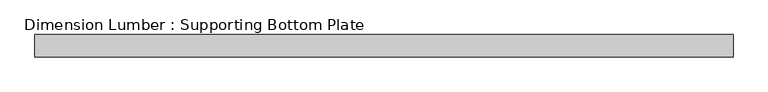
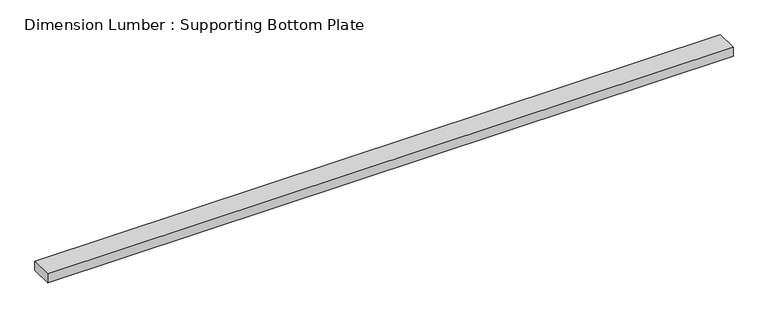
"""IFC4 building model written with IfcOpenShell, lengths in millimetres: beam geometry, Dimension Lumber : Supporting Bottom Plate."""

from ifc_helpers import new_model, si_unit, frame, origin, place, context, project, spatial, polyline, outline, extrude, source, transform, mapped, element, save


def dimension_lumber_supporting_bottom_plate_ae810c3f(model_context):
    return source(origin(), model_context, "Body", "SweptSolid", [
        extrude(outline(polyline([(1404.540625, 44.45), (1404.540625, -44.45), (-1385.490625, -44.45), (-1385.490625, 44.45), (1404.540625, 44.45)])), frame((0.0, 0.0, -19.05), z_axis=(0.0, 0.0, 1.0), x_axis=(1.0, 0.0, 0.0)), (0.0, 0.0, 1.0), 38.1),
    ])


if __name__ == "__main__":
    model = new_model("IFC4")
    model_context = context("Model", 3, world=origin())
    ifc_project = project(units=[si_unit("LENGTHUNIT", "METRE", prefix="MILLI")], contexts=[model_context])
    site = spatial("IfcSite", under=ifc_project)
    building = spatial("IfcBuilding", under=site)
    placement = place(None, origin())
    dimension_lumber_supporting_bottom_plate_shape = dimension_lumber_supporting_bottom_plate_ae810c3f(model_context)
    element("IfcBeam", 1, ObjectType="Dimension Lumber : Supporting Bottom Plate", at=placement, inside=building, context=model_context, shape_type="MappedRepresentation", body=[
        mapped(dimension_lumber_supporting_bottom_plate_shape, transform((0.0, 0.0, 0.0), x_axis=(1.0, 0.0, 0.0), y_axis=(0.0, 1.0, 0.0), z_axis=(0.0, 0.0, 1.0))),
    ])
    save(model, "model.ifc")

# Revit data of these elements
# Type "Dimension Lumber : Supporting Bottom Plate"
#   Assembly Code = "B10"
#   A = 0.0364583 SF
#   Length [instance default] = 5' - 0"
#   b = 0' - 3 1/2"
#   d = 0' - 1 1/2"
#   Structural Material [instance default] = Softwood, Lumber
# Element 1 (IfcBeam, "Dimension Lumber : Supporting Bottom Plate")
#   Structural Material = Douglas Fir #2
#   Materials on its faces: "Douglas Fir #2"
# Materials
#   "Softwood, Lumber": class "Wood", colour RGB 223 192 134, transparency 0, Description = "Pinus Echinata", Cost = 0
#   "Douglas Fir #2": class "Wood", colour RGB 223 192 134, transparency 0, Description = "Pinus Echinata", Cost = 0
